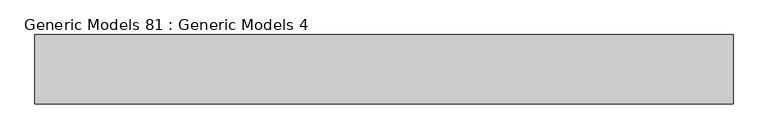
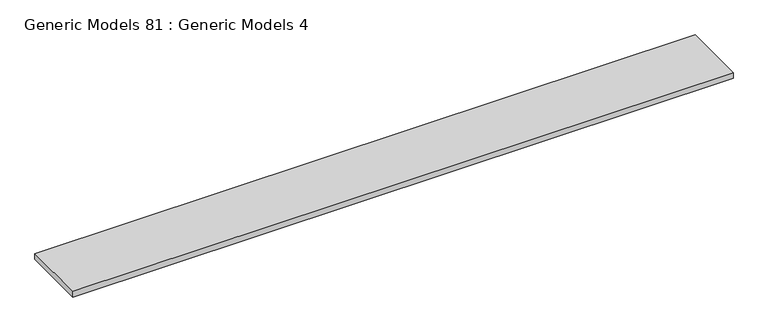
"""IFC4 building model written with IfcOpenShell, lengths in millimetres: proxy geometry, Generic Models 81 : Generic Models 4."""

from ifc_helpers import new_model, si_unit, frame, origin, place, context, project, spatial, polyline, outline, extrude, source, transform, mapped, element, save


def generic_models_81_generic_models_4_9d59f18e(model_context):
    return source(origin(), model_context, "Body", "SweptSolid", [
        extrude(outline(polyline([(28652.0604162, -7352.2318256), (28652.0604162, -7897.898997), (23168.0573109, -7897.898997), (23168.0573109, -7352.2318256), (28652.0604162, -7352.2318256)])), frame((0.0, 0.0, 123157.996), z_axis=(0.0, 0.0, 1.0), x_axis=(1.0, 0.0, 0.0)), (0.0, 0.0, 1.0), 50.8),
    ])


if __name__ == "__main__":
    model = new_model("IFC4")
    model_context = context("Model", 3, world=origin())
    ifc_project = project(units=[si_unit("LENGTHUNIT", "METRE", prefix="MILLI")], contexts=[model_context])
    site = spatial("IfcSite", under=ifc_project)
    building = spatial("IfcBuilding", under=site)
    placement = place(None, origin())
    generic_models_81_generic_models_4_shape = generic_models_81_generic_models_4_9d59f18e(model_context)
    element("IfcBuildingElementProxy", 1, Name="Generic Models 81 : Generic Models 4", ObjectType="Generic Models 81 : Generic Models 4", at=placement, inside=building, context=model_context, shape_type="MappedRepresentation", body=[
        mapped(generic_models_81_generic_models_4_shape, transform((0.0, 0.0, 0.0), x_axis=(1.0, 0.0, 0.0), y_axis=(0.0, 1.0, 0.0), z_axis=(0.0, 0.0, 1.0))),
    ])
    save(model, "model.ifc")

# Revit data of these elements
# Element 1 (IfcBuildingElementProxy, "Generic Models 81 : Generic Models 4")
#   Materials on its faces: "_2\" SAND"
# Materials
#   "_2\" SAND": class "Generic", colour RGB 245 226 173, transparency 0, Cost = 0
